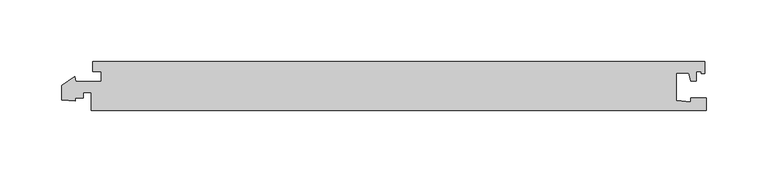
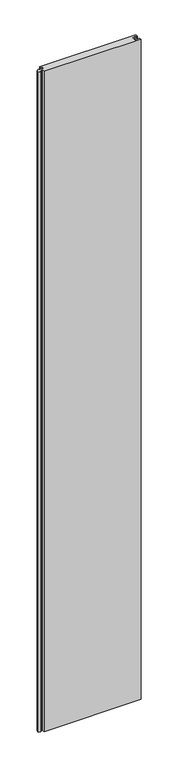
"""IFC4 building model written with IfcOpenShell, lengths in millimetres: proxy geometry, Generic Models 5:Generic Models 5:321804:Generic Models 5:321804 : Generic Models 5:Generic Models 5:321804:30 : Generic Models 5:Generic Models 5:321804:Generic Models 5:321804 : Generic Models 5:Generic Models 5:321804:300761."""

from ifc_helpers import new_model, si_unit, frame, origin, place, context, project, spatial, polyline, outline, extrude, source, transform, mapped, element, save


def generic_models_d8c8442d(model_context):
    return source(origin(), model_context, "Body", "SweptSolid", [
        extrude(outline(polyline([(593294.8386129, -568238.0537319), (593284.4802827, -568238.0537319), (593284.4802827, -568260.5495221), (593296.4802827, -568261.5993861), (593296.4802827, -568258.3537319), (593309.2302827, -568258.3537319), (593309.2302827, -568268.5537319), (592809.2302827, -568268.5537319), (592809.2302827, -568254.0537319), (592802.6052827, -568254.0537319), (592802.6052827, -568258.3537319), (592795.9802827, -568258.3537319), (592795.9802827, -568261.0537319), (592784.9802827, -568260.0913566), (592784.9802827, -568248.2332156), (592795.6617846, -568241.1258504), (592796.7142572, -568245.0537319), (592817.4302827, -568245.0537319), (592817.4302827, -568237.0537319), (592810.4802827, -568237.0537319), (592810.4802827, -568228.5537319), (593307.9802827, -568228.5537319), (593307.9802827, -568238.5537319), (593304.9802827, -568238.5537319), (593304.9802827, -568237.0537319), (593301.0302827, -568237.0537319), (593301.0302827, -568244.5537319), (593296.5802827, -568244.5537319), (593294.8386129, -568238.0537319)])), frame((0.0, 0.0, 4922.3046696), z_axis=(0.0, 0.0, 1.0), x_axis=(1.0, 0.0, 0.0)), (0.0, 0.0, 1.0), 3596.3565073),
    ])


if __name__ == "__main__":
    model = new_model("IFC4")
    model_context = context("Model", 3, world=origin())
    ifc_project = project(units=[si_unit("LENGTHUNIT", "METRE", prefix="MILLI")], contexts=[model_context])
    site = spatial("IfcSite", under=ifc_project)
    building = spatial("IfcBuilding", under=site)
    placement = place(None, origin())
    generic_models_shape = generic_models_d8c8442d(model_context)
    element("IfcBuildingElementProxy", 1, Name="Generic Models 5:Generic Models 5:321804:Generic Models 5:321804 : Generic Models 5:Generic Models 5:321804:30 : Generic Models 5:Generic Models 5:321804:Generic Models 5:321804 : Generic Models 5:Generic Models 5:321804:300761", ObjectType="Generic Models 5:Generic Models 5:321804:Generic Models 5:321804 : Generic Models 5:Generic Models 5:321804:30 : Generic Models 5:Generic Models 5:321804:Generic Models 5:321804 : Generic Models 5:Generic Models 5:321804:300761", at=placement, inside=building, context=model_context, shape_type="MappedRepresentation", body=[
        mapped(generic_models_shape, transform((0.0, 0.0, 0.0), x_axis=(1.0, 0.0, 0.0), y_axis=(0.0, 1.0, 0.0), z_axis=(0.0, 0.0, 1.0))),
    ])
    save(model, "model.ifc")

# Revit data of these elements
# Type "Generic Models 5:Generic Models 5:321804:Generic Models 5:321804 : Generic Models 5:Generic Models 5:321804:30 : Generic Models 5:Generic Models 5:321804:Generic Models 5:321804 : Generic Models 5:Generic Models 5:321804:300761"
#   NameOverride = "Generic Models 5:Generic Models 5:321804:Generic Models 5:321804 : Generic Models 5:Generic Models 5:321804:300761"
#   ObjectTypeOverride = "Generic Models 5:321804 : Generic Models 5:Generic Models 5:321804"
#   Reference = "Generic Models 5"
#   Tag = "300761"
# Element 1 (IfcBuildingElementProxy, "Generic Models 5:Generic Models 5:321804:Generic Models 5:321804 : Generic Models 5:Generic Models 5:321804:30 : Generic Models 5:Generic Models 5:321804:Generic Models 5:321804 : Generic Models 5:Generic Models 5:321804:300761")
#   Materials on its faces: "POLYCARBONATE PANEL - ARCOPLUS 547"
# Materials
#   "POLYCARBONATE PANEL - ARCOPLUS 547": class "Unassigned", colour RGB 202 225 249, transparency 0.45, Cost = 0
